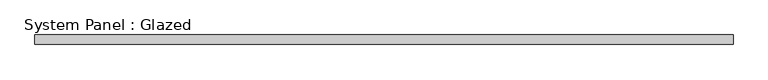
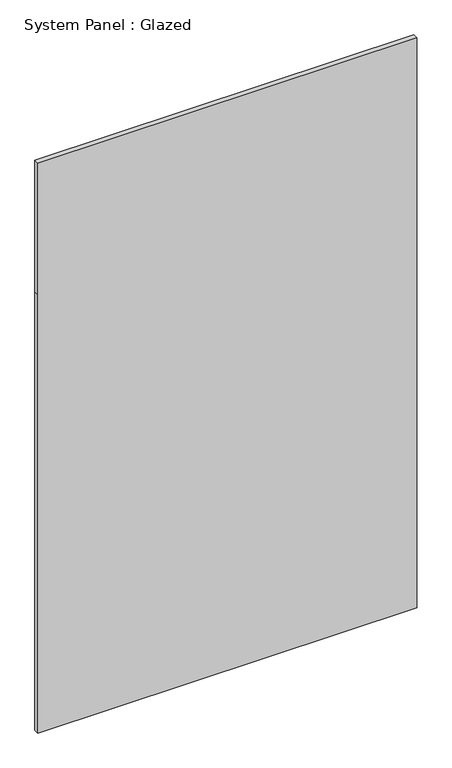
"""IFC4 building model written with IfcOpenShell, lengths in millimetres: plate geometry, System Panel : Glazed."""

import ifcopenshell
import ifcopenshell.guid

model = None  # the IFC model being written
_history = None  # IfcOwnerHistory: only IFC2X3 demands one
_inside = {}  # id of a spatial element -> (the spatial element, [elements in it])
_under = {}  # id of a project, library or spatial element -> (it, [spatial elements below it])
_declared = {}  # id of a project -> (the project, [libraries it declares])
_typed = {}  # id of a type object -> (the type object, [elements of that type])
_made_of = {}  # id of a material, layer set ... -> (it, [elements and type objects made of it])


def new_model(schema):
    """Start an empty IFC model of exactly this schema.

    Asked for "IFC4X3", IfcOpenShell would pick the latest addendum, in which some entities
    have other attributes; the version numbers below select the first issue.
    IFC2X3 requires an IfcOwnerHistory on every rooted entity: one is made here for all.
    """
    global model, _history
    if schema == "IFC4X3":
        model = ifcopenshell.file(schema_version=(4, 3, 0, 0))
    else:
        model = ifcopenshell.file(schema=schema)
    _inside.clear()
    _under.clear()
    _declared.clear()
    _typed.clear()
    _made_of.clear()
    _history = None
    if model.schema == "IFC2X3":
        org = make("IfcOrganization", Name="unknown")
        user = make(
            "IfcPersonAndOrganization",
            ThePerson=make("IfcPerson", FamilyName="unknown"),
            TheOrganization=org,
        )
        app = make(
            "IfcApplication",
            ApplicationDeveloper=org,
            Version="unknown",
            ApplicationFullName="unknown",
            ApplicationIdentifier="unknown",
        )
        _history = make(
            "IfcOwnerHistory",
            OwningUser=user,
            OwningApplication=app,
            ChangeAction="ADDED",
            CreationDate=0,
        )
    return model


def make(cls, **values):
    """One entity of the class cls with the attributes given. An attribute that is None is left unset."""
    return model.create_entity(
        cls, **{name: value for name, value in values.items() if value is not None}
    )


def rooted(cls, **values):
    """An entity with a GlobalId (a new one), such as an element, a storey or a relation."""
    return make(cls, GlobalId=ifcopenshell.guid.new(), OwnerHistory=_history, **values)


def si_unit(unit_type, name, prefix=None):
    """IfcSIUnit, for example si_unit("LENGTHUNIT", "METRE", prefix="MILLI")."""
    return make("IfcSIUnit", UnitType=unit_type, Prefix=prefix, Name=name)


def assignment(units):
    """IfcUnitAssignment: the units of a project."""
    return None if units is None else make("IfcUnitAssignment", Units=units)


def point(xyz):
    """IfcCartesianPoint."""
    return None if xyz is None else make("IfcCartesianPoint", Coordinates=xyz)


def direction(xyz):
    """IfcDirection."""
    return None if xyz is None else make("IfcDirection", DirectionRatios=xyz)


def frame(location, z_axis=None, x_axis=None):
    """IfcAxis2Placement3D, a coordinate frame: its origin and axes. An axis left out is left unset."""
    return make(
        "IfcAxis2Placement3D",
        Location=point(location),
        Axis=direction(z_axis),
        RefDirection=direction(x_axis),
    )


def origin():
    """The frame at (0, 0, 0) with its axes left unset."""
    return frame((0.0, 0.0, 0.0))


def place(relative_to, where):
    """IfcLocalPlacement: puts the frame where relative to a parent placement (None: the world)."""
    return make(
        "IfcLocalPlacement", PlacementRelTo=relative_to, RelativePlacement=where
    )


def context(
    kind, dimensions, precision=None, world=None, true_north=None, identifier=None
):
    """IfcGeometricRepresentationContext, for example the 3D "Model" context."""
    return make(
        "IfcGeometricRepresentationContext",
        ContextIdentifier=identifier,
        ContextType=kind,
        CoordinateSpaceDimension=dimensions,
        Precision=precision,
        WorldCoordinateSystem=world,
        TrueNorth=true_north,
    )


def project(units=None, contexts=None):
    """IfcProject with its units and contexts."""
    return rooted(
        "IfcProject",
        Name="project",
        RepresentationContexts=contexts,
        UnitsInContext=assignment(units),
    )


def spatial(cls, under=None, at=None, **own):
    """A site, building, storey or space (cls), placed at a placement, below another one or the project."""
    s = rooted(cls, ObjectPlacement=at, **own)
    if under is not None:
        _under.setdefault(under.id(), (under, []))[1].append(s)
    return s


def polyline(points):
    """IfcPolyline through the points."""
    return make("IfcPolyline", Points=[point(p) for p in points])


def outline(outer, holes=None, kind="AREA"):
    """IfcArbitraryClosedProfileDef: a profile drawn as a closed curve; with holes, ...WithVoids."""
    if holes is None:
        return make("IfcArbitraryClosedProfileDef", ProfileType=kind, OuterCurve=outer)
    return make(
        "IfcArbitraryProfileDefWithVoids",
        ProfileType=kind,
        OuterCurve=outer,
        InnerCurves=holes,
    )


def extrude(swept, where, along, depth):
    """IfcExtrudedAreaSolid: the profile swept, set in the frame where, extruded along a direction by depth."""
    return make(
        "IfcExtrudedAreaSolid",
        SweptArea=swept,
        Position=where,
        ExtrudedDirection=direction(along),
        Depth=depth,
    )


def shape(context_of_items, identifier, shape_type, items):
    """IfcShapeRepresentation: the items that make up one representation, for example the "Body"."""
    return make(
        "IfcShapeRepresentation",
        ContextOfItems=context_of_items,
        RepresentationIdentifier=identifier,
        RepresentationType=shape_type,
        Items=items,
    )


def source(mapping_origin, context_of_items, identifier, shape_type, items):
    """IfcRepresentationMap: a shape defined once, which mapped items show again and again."""
    return make(
        "IfcRepresentationMap",
        MappingOrigin=mapping_origin,
        MappedRepresentation=shape(context_of_items, identifier, shape_type, items),
    )


def transform(
    local_origin,
    x_axis=None,
    y_axis=None,
    z_axis=None,
    scale=None,
    scale2=None,
    scale3=None,
    uniform=True,
):
    """IfcCartesianTransformationOperator3D, or its non-uniform kind. x_axis, y_axis, z_axis: its Axis1, 2, 3."""
    if uniform:
        return make(
            "IfcCartesianTransformationOperator3D",
            Axis1=direction(x_axis),
            Axis2=direction(y_axis),
            LocalOrigin=point(local_origin),
            Scale=scale,
            Axis3=direction(z_axis),
        )
    return make(
        "IfcCartesianTransformationOperator3DnonUniform",
        Axis1=direction(x_axis),
        Axis2=direction(y_axis),
        LocalOrigin=point(local_origin),
        Scale=scale,
        Axis3=direction(z_axis),
        Scale2=scale2,
        Scale3=scale3,
    )


def mapped(mapping_source, mapping_target):
    """IfcMappedItem: shows the shape of a source again, moved by a transform."""
    return make(
        "IfcMappedItem", MappingSource=mapping_source, MappingTarget=mapping_target
    )


def made_of(thing, what):
    """Note that an element or type object is made of a material, layer set ...; save() writes the relation."""
    if what is not None:
        _made_of.setdefault(what.id(), (what, []))[1].append(thing)
    return thing


def element(
    cls,
    number,
    at=None,
    inside=None,
    cuts=None,
    type_object=None,
    material=None,
    context=None,
    identifier="Body",
    shape_type=None,
    held_by="IfcProductDefinitionShape",
    body=None,
    shapes=None,
    **own,
):
    """One element of the class cls, such as IfcWall. Its Tag is "e" and its number.

    at: its placement. inside: the storey or other place that contains it. cuts: it is an
    opening in that element (IfcRelVoidsElement). A single representation is given by context,
    identifier, shape_type and body (its items); several are given by shapes. held_by: the class
    of the entity that holds the representations. save() writes the other relations.
    """
    e = rooted(cls, Tag="e%d" % number, ObjectPlacement=at, **own)
    if body is not None:
        shapes = [shape(context, identifier, shape_type, body)]
    if shapes is not None:
        e.Representation = make(held_by, Representations=shapes)
    if inside is not None:
        _inside.setdefault(inside.id(), (inside, []))[1].append(e)
    if cuts is not None:
        rooted(
            "IfcRelVoidsElement", RelatingBuildingElement=cuts, RelatedOpeningElement=e
        )
    if type_object is not None:
        _typed.setdefault(type_object.id(), (type_object, []))[1].append(e)
    return made_of(e, material)


def aggregate(whole, parts):
    """IfcRelAggregates: a whole, such as a stair, and the parts it consists of."""
    return rooted("IfcRelAggregates", RelatingObject=whole, RelatedObjects=parts)


def save(model, path):
    """Write the relations noted so far, then the file.

    IfcRelAggregates (storeys below a building ...), IfcRelContainedInSpatialStructure (elements
    in a storey), IfcRelDefinesByType, IfcRelAssociatesMaterial and IfcRelDeclares: one each for
    every whole, place, type object, material and project.
    """
    for whole, parts in _under.values():
        aggregate(whole, parts)
    for where, things in _inside.values():
        rooted(
            "IfcRelContainedInSpatialStructure",
            RelatedElements=things,
            RelatingStructure=where,
        )
    for kind, things in _typed.values():
        rooted("IfcRelDefinesByType", RelatedObjects=things, RelatingType=kind)
    for what, things in _made_of.values():
        rooted("IfcRelAssociatesMaterial", RelatedObjects=things, RelatingMaterial=what)
    for by, libraries in _declared.values():
        rooted("IfcRelDeclares", RelatingContext=by, RelatedDefinitions=libraries)
    model.write(path)


def system_panel_glazed_242ba3c9(model_context):
    return source(origin(), model_context, "Body", "SweptSolid", [
        extrude(outline(polyline([(0.0, -919.4444444), (0.0, 919.4444444), (2250.0, 919.4444444), (2925.0, 919.4444444), (2925.0, -919.4444444), (2250.0, -919.4444444), (0.0, -919.4444444)])), frame((0.0, 24.5, 0.0), z_axis=(0.0, 1.0, 0.0), x_axis=(0.0, 0.0, 1.0)), (0.0, 0.0, 1.0), 25.0),
    ])


if __name__ == "__main__":
    model = new_model("IFC4")
    model_context = context("Model", 3, world=origin())
    ifc_project = project(units=[si_unit("LENGTHUNIT", "METRE", prefix="MILLI")], contexts=[model_context])
    site = spatial("IfcSite", under=ifc_project)
    building = spatial("IfcBuilding", under=site)
    placement = place(None, origin())
    system_panel_glazed_shape = system_panel_glazed_242ba3c9(model_context)
    element("IfcPlate", 1, ObjectType="System Panel : Glazed", at=placement, inside=building, context=model_context, shape_type="MappedRepresentation", body=[
        mapped(system_panel_glazed_shape, transform((0.0, 0.0, 0.0), x_axis=(1.0, 0.0, 0.0), y_axis=(0.0, 1.0, 0.0), z_axis=(0.0, 0.0, 1.0))),
    ])
    save(model, "model.ifc")

# Revit data of these elements
# Element 1 (IfcPlate, "System Panel : Glazed")
#   Materials on its faces: "Glass"
# Materials
#   "Glass": class "Glass", colour RGB 0 128 192, transparency 0.9
